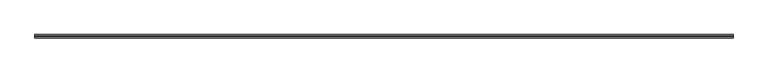
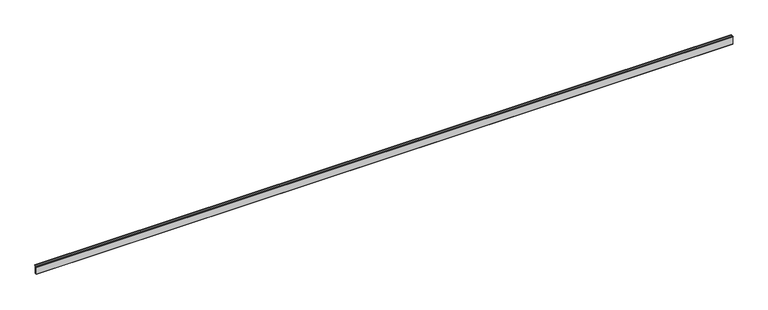
"""IFC4 building model written with IfcOpenShell, lengths in millimetres: railing geometry, ML_Perfil U de embutir : ML_Perfil U de embutir."""

from ifc_helpers import new_model, si_unit, frame, origin, place, context, project, spatial, polyline, outline, extrude, source, transform, mapped, element, save


def railing_3a0e213f(model_context):
    return source(origin(), model_context, "Body", "SweptSolid", [
        extrude(outline(polyline([(1832.4523952, 3702.0), (1832.4523952, 3594.0), (1856.4523952, 3594.0), (1856.4523952, 3702.0), (1866.9523952, 3702.0), (1866.9523952, 3700.0), (1858.4523952, 3700.0), (1858.4523952, 3592.0), (1830.4523952, 3592.0), (1830.4523952, 3700.0), (1821.9523952, 3700.0), (1821.9523952, 3702.0), (1832.4523952, 3702.0)])), frame((-12226.1487231, 0.0, 0.0), z_axis=(1.0, 0.0, 0.0), x_axis=(0.0, 1.0, 0.0)), (0.0, 0.0, 1.0), 9335.0),
    ])


if __name__ == "__main__":
    model = new_model("IFC4")
    model_context = context("Model", 3, world=origin())
    ifc_project = project(units=[si_unit("LENGTHUNIT", "METRE", prefix="MILLI")], contexts=[model_context])
    site = spatial("IfcSite", under=ifc_project)
    building = spatial("IfcBuilding", under=site)
    placement = place(None, origin())
    railing_shape = railing_3a0e213f(model_context)
    element("IfcRailing", 1, ObjectType="ML_Perfil U de embutir : ML_Perfil U de embutir", at=placement, inside=building, context=model_context, shape_type="MappedRepresentation", body=[
        mapped(railing_shape, transform((0.0, 0.0, 0.0), x_axis=(1.0, 0.0, 0.0), y_axis=(0.0, 1.0, 0.0), z_axis=(0.0, 0.0, 1.0))),
    ])
    save(model, "model.ifc")

# Revit data of these elements
# Type "ML_Perfil U de embutir : ML_Perfil U de embutir"
#   ME_Compr [instance default] = 9.335 m
#   ME_Material Perfil [instance default] = .ALUMÍNIO COM PINTURA ELETROSTÁTICA BRANCA
# Element 1 (IfcRailing, "ML_Perfil U de embutir : ML_Perfil U de embutir")
#   Materials on its faces: ".ALUMÍNIO COM PINTURA ELETROSTÁTICA BRANCA"
# Materials
#   ".ALUMÍNIO COM PINTURA ELETROSTÁTICA BRANCA": class "CC_METAIS", colour RGB 241 241 241, transparency 0, Cost = 0
